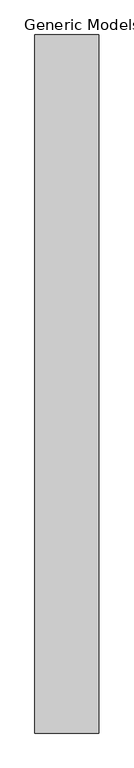
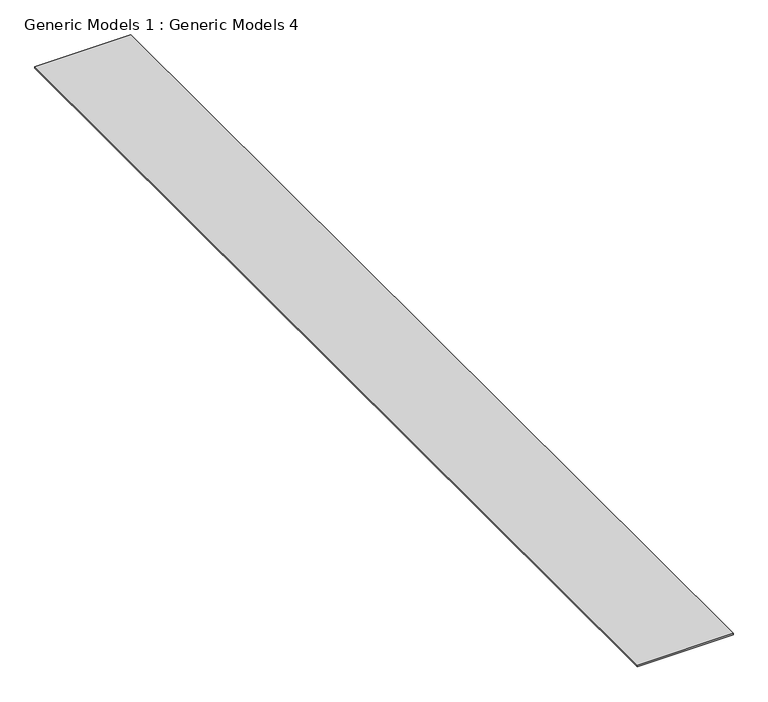
"""IFC4 building model written with IfcOpenShell, lengths in millimetres: proxy geometry, Generic Models 1 : Generic Models 4."""

from ifc_helpers import new_model, si_unit, frame, origin, place, context, project, spatial, polyline, outline, extrude, source, transform, mapped, element, save


def generic_models_1_generic_models_4_e06103ed(model_context):
    return source(origin(), model_context, "Body", "SweptSolid", [
        extrude(outline(polyline([(8397.5835152, -464.1230338), (7273.8692257, -464.1230338), (7273.8692257, 11778.6769662), (8397.5835152, 11778.6769662), (8397.5835152, -464.1230338)])), frame((0.0, 0.0, 126364.746), z_axis=(0.0, 0.0, 1.0), x_axis=(1.0, 0.0, 0.0)), (0.0, 0.0, 1.0), 19.05),
    ])


if __name__ == "__main__":
    model = new_model("IFC4")
    model_context = context("Model", 3, world=origin())
    ifc_project = project(units=[si_unit("LENGTHUNIT", "METRE", prefix="MILLI")], contexts=[model_context])
    site = spatial("IfcSite", under=ifc_project)
    building = spatial("IfcBuilding", under=site)
    placement = place(None, origin())
    generic_models_1_generic_models_4_shape = generic_models_1_generic_models_4_e06103ed(model_context)
    element("IfcBuildingElementProxy", 1, Name="Generic Models 1 : Generic Models 4", ObjectType="Generic Models 1 : Generic Models 4", at=placement, inside=building, context=model_context, shape_type="MappedRepresentation", body=[
        mapped(generic_models_1_generic_models_4_shape, transform((0.0, 0.0, 0.0), x_axis=(1.0, 0.0, 0.0), y_axis=(0.0, 1.0, 0.0), z_axis=(0.0, 0.0, 1.0))),
    ])
    save(model, "model.ifc")

# Revit data of these elements
# Element 1 (IfcBuildingElementProxy, "Generic Models 1 : Generic Models 4")
#   Materials on its faces: "FIRE RETARDANT TREATED WOOD SOFFIT"
# Materials
#   "FIRE RETARDANT TREATED WOOD SOFFIT": class "Generic", colour RGB 177 130 114, transparency 0, Cost = 0
